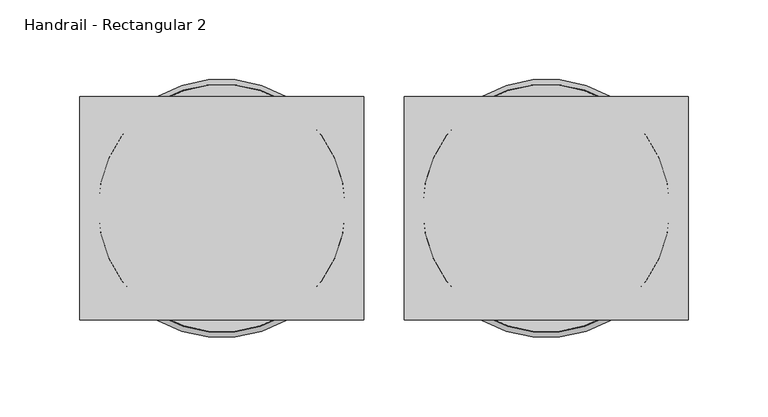
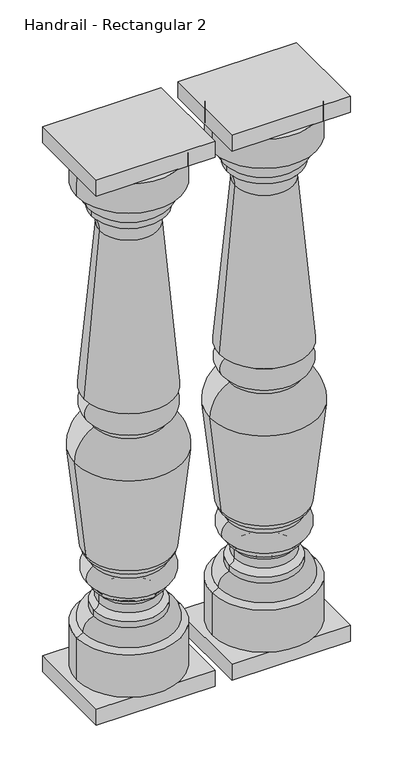
"""IFC4 building model written with IfcOpenShell, lengths in millimetres: railing geometry, Handrail - Rectangular 2."""

from ifc_helpers import new_model, si_unit, point, frame, origin, place, context, project, spatial, polyline, circle_curve, ellipse_curve, trimmed, outline, extrude, source, transform, mapped, element, save
from ifc_brep_helpers import plane_surface, cylinder_surface, revolved_surface, advanced_brep


def handrail_rectangular_2_7eab9a82(model_context):
    return source(origin(), model_context, "Body", "SolidModel", [
        advanced_brep(
        [(9255.6521895, -1691.0164768, 949.325), (9178.0909506, -1691.0164768, 949.325), (9333.2134284, -1691.0164768, 949.325), (9333.4396895, -1691.0164768, 136.525), (9177.8646895, -1691.0164768, 136.525), (9255.6521895, -1691.0164768, 136.525), (9333.4396895, -1691.0164768, 203.2), (9177.8646895, -1691.0164768, 203.2), (9323.8276556, -1691.0164768, 208.348485), (9187.4767235, -1691.0164768, 208.348485), (9308.0396895, -1691.0164768, 228.7310532), (9203.2646895, -1691.0164768, 228.7310532), (9308.0396895, -1691.0164768, 238.125), (9203.2646895, -1691.0164768, 238.125), (9300.4209727, -1691.0164768, 247.1598162), (9210.8834064, -1691.0164768, 247.1598162), (9300.4209727, -1691.0164768, 260.8401838), (9210.8834064, -1691.0164768, 260.8401838), (9308.0396895, -1691.0164768, 269.875), (9203.2646895, -1691.0164768, 269.875), (9308.0396895, -1691.0164768, 276.225), (9203.2646895, -1691.0164768, 276.225), (9308.8334395, -1691.0164768, 307.975), (9202.4709395, -1691.0164768, 307.975), (9308.8334395, -1691.0164768, 314.325), (9202.4709395, -1691.0164768, 314.325), (9319.6062243, -1691.0164768, 327.0157842), (9191.6981547, -1691.0164768, 327.0157842), (9336.693305, -1691.0164768, 481.3725887), (9174.6110741, -1691.0164768, 481.3725887), (9308.0396895, -1691.0164768, 528.6375), (9203.2646895, -1691.0164768, 528.6375), (9308.0396895, -1691.0164768, 534.9875), (9203.2646895, -1691.0164768, 534.9875), (9311.2146895, -1691.0164768, 569.9125), (9200.0896895, -1691.0164768, 569.9125), (9311.2146895, -1691.0164768, 573.0875), (9200.0896895, -1691.0164768, 573.0875), (9322.3271895, -1691.0164768, 577.85), (9188.9771895, -1691.0164768, 577.85), (9299.1486775, -1691.0164768, 836.3199218), (9212.1557016, -1691.0164768, 836.3199218), (9311.2146895, -1691.0164768, 863.6), (9200.0896895, -1691.0164768, 863.6), (9311.2146895, -1691.0164768, 873.125), (9200.0896895, -1691.0164768, 873.125), (9322.3271895, -1691.0164768, 900.1125), (9188.9771895, -1691.0164768, 900.1125), (9333.4396895, -1691.0164768, 903.2875), (9177.8646895, -1691.0164768, 903.2875)],
        [
            (0, 1),
            (1, 2, circle_curve(frame((9255.6521895, -1691.0164768, 949.325), z_axis=(0.0, 0.0, 1.0), x_axis=(-1.0, 0.0, 0.0)), 77.5612389)),
            (2, 0),
            (2, 1, circle_curve(frame((9255.6521895, -1691.0164768, 949.325), z_axis=(0.0, 0.0, 1.0), x_axis=(-1.0, 0.0, 0.0)), 77.5612389)),
            (3, 4, circle_curve(frame((9255.6521895, -1691.0164768, 136.525), z_axis=(0.0, 0.0, -1.0), x_axis=(-1.0, 0.0, 0.0)), 77.7875)),
            (4, 5),
            (5, 3),
            (4, 3, circle_curve(frame((9255.6521895, -1691.0164768, 136.525), z_axis=(0.0, 0.0, -1.0), x_axis=(-1.0, 0.0, 0.0)), 77.7875)),
            (6, 7, circle_curve(frame((9255.6521895, -1691.0164768, 203.2), z_axis=(0.0, 0.0, -1.0), x_axis=(-1.0, 0.0, 0.0)), 77.7875)),
            (7, 4),
            (3, 6),
            (7, 6, circle_curve(frame((9255.6521895, -1691.0164768, 203.2), z_axis=(0.0, 0.0, -1.0), x_axis=(-1.0, 0.0, 0.0)), 77.7875)),
            (8, 9, circle_curve(frame((9255.6521895, -1691.0164768, 208.348485), z_axis=(0.0, 0.0, -1.0), x_axis=(-1.0, 0.0, 0.0)), 68.175466)),
            (9, 7),
            (6, 8),
            (9, 8, circle_curve(frame((9255.6521895, -1691.0164768, 208.348485), z_axis=(0.0, 0.0, -1.0), x_axis=(-1.0, 0.0, 0.0)), 68.175466)),
            (10, 11, circle_curve(frame((9255.6521895, -1691.0164768, 228.7310532), z_axis=(0.0, 0.0, -1.0), x_axis=(-1.0, 0.0, 0.0)), 52.3875)),
            (11, 9, circle_curve(frame((9205.6397784, -1691.0164768, 210.5855331), z_axis=(0.0, -1.0, 0.0), x_axis=(1.0, 0.0, 0.0)), 18.3002991)),
            (8, 10, circle_curve(frame((9305.6646007, -1691.0164768, 210.5855331), z_axis=(0.0, -1.0, 0.0), x_axis=(-1.0, 0.0, 0.0)), 18.3002991)),
            (11, 10, circle_curve(frame((9255.6521895, -1691.0164768, 228.7310532), z_axis=(0.0, 0.0, -1.0), x_axis=(-1.0, 0.0, 0.0)), 52.3875)),
            (12, 13, circle_curve(frame((9255.6521895, -1691.0164768, 238.125), z_axis=(0.0, 0.0, -1.0), x_axis=(-1.0, 0.0, 0.0)), 52.3875)),
            (13, 11),
            (10, 12),
            (13, 12, circle_curve(frame((9255.6521895, -1691.0164768, 238.125), z_axis=(0.0, 0.0, -1.0), x_axis=(-1.0, 0.0, 0.0)), 52.3875)),
            (14, 15, circle_curve(frame((9255.6521895, -1691.0164768, 247.1598162), z_axis=(0.0, 0.0, -1.0), x_axis=(-1.0, 0.0, 0.0)), 44.7687831)),
            (15, 13, circle_curve(frame((9201.4793543, -1691.0164768, 247.3602005), z_axis=(0.0, 1.0, 0.0), x_axis=(1.0, 0.0, 0.0)), 9.4061868)),
            (12, 14, circle_curve(frame((9309.8250248, -1691.0164768, 247.3602005), z_axis=(0.0, 1.0, 0.0), x_axis=(-1.0, 0.0, 0.0)), 9.4061868)),
            (15, 14, circle_curve(frame((9255.6521895, -1691.0164768, 247.1598162), z_axis=(0.0, 0.0, -1.0), x_axis=(-1.0, 0.0, 0.0)), 44.7687831)),
            (16, 17, circle_curve(frame((9255.6521895, -1691.0164768, 260.8401838), z_axis=(0.0, 0.0, -1.0), x_axis=(-1.0, 0.0, 0.0)), 44.7687831)),
            (17, 15),
            (14, 16),
            (17, 16, circle_curve(frame((9255.6521895, -1691.0164768, 260.8401838), z_axis=(0.0, 0.0, -1.0), x_axis=(-1.0, 0.0, 0.0)), 44.7687831)),
            (18, 19, circle_curve(frame((9255.6521895, -1691.0164768, 269.875), z_axis=(0.0, 0.0, -1.0), x_axis=(-1.0, 0.0, 0.0)), 52.3875)),
            (19, 17, circle_curve(frame((9201.4793543, -1691.0164768, 260.6397995), z_axis=(0.0, 1.0, 0.0), x_axis=(1.0, 0.0, 0.0)), 9.4061868)),
            (16, 18, circle_curve(frame((9309.8250248, -1691.0164768, 260.6397995), z_axis=(0.0, 1.0, 0.0), x_axis=(-1.0, 0.0, 0.0)), 9.4061868)),
            (19, 18, circle_curve(frame((9255.6521895, -1691.0164768, 269.875), z_axis=(0.0, 0.0, -1.0), x_axis=(-1.0, 0.0, 0.0)), 52.3875)),
            (20, 21, circle_curve(frame((9255.6521895, -1691.0164768, 276.225), z_axis=(0.0, 0.0, -1.0), x_axis=(-1.0, 0.0, 0.0)), 52.3875)),
            (21, 19),
            (18, 20),
            (21, 20, circle_curve(frame((9255.6521895, -1691.0164768, 276.225), z_axis=(0.0, 0.0, -1.0), x_axis=(-1.0, 0.0, 0.0)), 52.3875)),
            (22, 23, circle_curve(frame((9255.6521895, -1691.0164768, 307.975), z_axis=(0.0, 0.0, -1.0), x_axis=(-1.0, 0.0, 0.0)), 53.18125)),
            (23, 21, circle_curve(frame((9208.8437772, -1691.0164768, 292.2493991), z_axis=(0.0, -1.0, 0.0), x_axis=(1.0, 0.0, 0.0)), 16.9678397)),
            (20, 22, circle_curve(frame((9302.4606019, -1691.0164768, 292.2493991), z_axis=(0.0, -1.0, 0.0), x_axis=(-1.0, 0.0, 0.0)), 16.9678397)),
            (23, 22, circle_curve(frame((9255.6521895, -1691.0164768, 307.975), z_axis=(0.0, 0.0, -1.0), x_axis=(-1.0, 0.0, 0.0)), 53.18125)),
            (24, 25, circle_curve(frame((9255.6521895, -1691.0164768, 314.325), z_axis=(0.0, 0.0, -1.0), x_axis=(-1.0, 0.0, 0.0)), 53.18125)),
            (25, 23),
            (22, 24),
            (25, 24, circle_curve(frame((9255.6521895, -1691.0164768, 314.325), z_axis=(0.0, 0.0, -1.0), x_axis=(-1.0, 0.0, 0.0)), 53.18125)),
            (26, 27, circle_curve(frame((9255.6521895, -1691.0164768, 327.0157842), z_axis=(0.0, 0.0, -1.0), x_axis=(-1.0, 0.0, 0.0)), 63.9540348)),
            (27, 25, circle_curve(frame((9212.304312, -1691.0164768, 333.5899445), z_axis=(0.0, -1.0, 0.0), x_axis=(1.0, 0.0, 0.0)), 21.6294545)),
            (24, 26, circle_curve(frame((9299.0000671, -1691.0164768, 333.5899445), z_axis=(0.0, -1.0, 0.0), x_axis=(-1.0, 0.0, 0.0)), 21.6294545)),
            (27, 26, circle_curve(frame((9255.6521895, -1691.0164768, 327.0157842), z_axis=(0.0, 0.0, -1.0), x_axis=(-1.0, 0.0, 0.0)), 63.9540348)),
            (28, 29, circle_curve(frame((9255.6521895, -1691.0164768, 481.3725887), z_axis=(0.0, 0.0, -1.0), x_axis=(-1.0, 0.0, 0.0)), 81.0411154)),
            (29, 27, circle_curve(frame((10668.9385198, -1691.0164768, 568.6683698), z_axis=(0.0, -1.0, 0.0), x_axis=(1.0, 0.0, 0.0)), 1496.8751012)),
            (26, 28, circle_curve(frame((7842.3658592, -1691.0164768, 568.6683698), z_axis=(0.0, -1.0, 0.0), x_axis=(-1.0, 0.0, 0.0)), 1496.8751012)),
            (29, 28, circle_curve(frame((9255.6521895, -1691.0164768, 481.3725887), z_axis=(0.0, 0.0, -1.0), x_axis=(-1.0, 0.0, 0.0)), 81.0411154)),
            (30, 31, circle_curve(frame((9255.6521895, -1691.0164768, 528.6375), z_axis=(0.0, 0.0, -1.0), x_axis=(-1.0, 0.0, 0.0)), 52.3875)),
            (31, 29, circle_curve(frame((9226.3638402, -1691.0164768, 482.3161407), z_axis=(0.0, -1.0, 0.0), x_axis=(1.0, 0.0, 0.0)), 51.7613668)),
            (28, 30, circle_curve(frame((9284.9405389, -1691.0164768, 482.3161407), z_axis=(0.0, -1.0, 0.0), x_axis=(-1.0, 0.0, 0.0)), 51.7613668)),
            (31, 30, circle_curve(frame((9255.6521895, -1691.0164768, 528.6375), z_axis=(0.0, 0.0, -1.0), x_axis=(-1.0, 0.0, 0.0)), 52.3875)),
            (32, 33, circle_curve(frame((9255.6521895, -1691.0164768, 534.9875), z_axis=(0.0, 0.0, -1.0), x_axis=(-1.0, 0.0, 0.0)), 52.3875)),
            (33, 31),
            (30, 32),
            (33, 32, circle_curve(frame((9255.6521895, -1691.0164768, 534.9875), z_axis=(0.0, 0.0, -1.0), x_axis=(-1.0, 0.0, 0.0)), 52.3875)),
            (34, 35, circle_curve(frame((9255.6521895, -1691.0164768, 569.9125), z_axis=(0.0, 0.0, -1.0), x_axis=(-1.0, 0.0, 0.0)), 55.5625)),
            (35, 33, circle_curve(frame((9208.3309419, -1691.0164768, 553.0548866), z_axis=(0.0, -1.0, 0.0), x_axis=(1.0, 0.0, 0.0)), 18.7642578)),
            (32, 34, circle_curve(frame((9302.9734372, -1691.0164768, 553.0548866), z_axis=(0.0, -1.0, 0.0), x_axis=(-1.0, 0.0, 0.0)), 18.7642578)),
            (35, 34, circle_curve(frame((9255.6521895, -1691.0164768, 569.9125), z_axis=(0.0, 0.0, -1.0), x_axis=(-1.0, 0.0, 0.0)), 55.5625)),
            (36, 37, circle_curve(frame((9255.6521895, -1691.0164768, 573.0875), z_axis=(0.0, 0.0, -1.0), x_axis=(-1.0, 0.0, 0.0)), 55.5625)),
            (37, 35),
            (34, 36),
            (37, 36, circle_curve(frame((9255.6521895, -1691.0164768, 573.0875), z_axis=(0.0, 0.0, -1.0), x_axis=(-1.0, 0.0, 0.0)), 55.5625)),
            (38, 39, circle_curve(frame((9255.6521895, -1691.0164768, 577.85), z_axis=(0.0, 0.0, -1.0), x_axis=(-1.0, 0.0, 0.0)), 66.675)),
            (39, 37),
            (36, 38),
            (39, 38, circle_curve(frame((9255.6521895, -1691.0164768, 577.85), z_axis=(0.0, 0.0, -1.0), x_axis=(-1.0, 0.0, 0.0)), 66.675)),
            (40, 41, circle_curve(frame((9255.6521895, -1691.0164768, 836.3199218), z_axis=(0.0, 0.0, -1.0), x_axis=(-1.0, 0.0, 0.0)), 43.4964879)),
            (41, 39, circle_curve(frame((7565.3192757, -1691.0164768, 853.7271544), z_axis=(0.0, 1.0, 0.0), x_axis=(1.0, 0.0, 0.0)), 1646.9284215)),
            (38, 40, circle_curve(frame((10945.9851034, -1691.0164768, 853.7271544), z_axis=(0.0, 1.0, 0.0), x_axis=(-1.0, 0.0, 0.0)), 1646.9284215)),
            (41, 40, circle_curve(frame((9255.6521895, -1691.0164768, 836.3199218), z_axis=(0.0, 0.0, -1.0), x_axis=(-1.0, 0.0, 0.0)), 43.4964879)),
            (42, 43, circle_curve(frame((9255.6521895, -1691.0164768, 863.6), z_axis=(0.0, 0.0, -1.0), x_axis=(-1.0, 0.0, 0.0)), 55.5625)),
            (43, 41, circle_curve(frame((9179.4515427, -1691.0164768, 838.1632773), z_axis=(0.0, 1.0, 0.0), x_axis=(1.0, 0.0, 0.0)), 32.7560676)),
            (40, 42, circle_curve(frame((9331.8528363, -1691.0164768, 838.1632773), z_axis=(0.0, 1.0, 0.0), x_axis=(-1.0, 0.0, 0.0)), 32.7560676)),
            (43, 42, circle_curve(frame((9255.6521895, -1691.0164768, 863.6), z_axis=(0.0, 0.0, -1.0), x_axis=(-1.0, 0.0, 0.0)), 55.5625)),
            (44, 45, circle_curve(frame((9255.6521895, -1691.0164768, 873.125), z_axis=(0.0, 0.0, -1.0), x_axis=(-1.0, 0.0, 0.0)), 55.5625)),
            (45, 43),
            (42, 44),
            (45, 44, circle_curve(frame((9255.6521895, -1691.0164768, 873.125), z_axis=(0.0, 0.0, -1.0), x_axis=(-1.0, 0.0, 0.0)), 55.5625)),
            (46, 47, circle_curve(frame((9255.6521895, -1691.0164768, 900.1125), z_axis=(0.0, 0.0, -1.0), x_axis=(-1.0, 0.0, 0.0)), 66.675)),
            (47, 45, circle_curve(frame((9218.3374113, -1691.0164768, 896.4203854), z_axis=(0.0, -1.0, 0.0), x_axis=(1.0, 0.0, 0.0)), 29.5914571)),
            (44, 46, circle_curve(frame((9292.9669678, -1691.0164768, 896.4203854), z_axis=(0.0, -1.0, 0.0), x_axis=(-1.0, 0.0, 0.0)), 29.5914571)),
            (47, 46, circle_curve(frame((9255.6521895, -1691.0164768, 900.1125), z_axis=(0.0, 0.0, -1.0), x_axis=(-1.0, 0.0, 0.0)), 66.675)),
            (48, 49, circle_curve(frame((9255.6521895, -1691.0164768, 903.2875), z_axis=(0.0, 0.0, -1.0), x_axis=(-1.0, 0.0, 0.0)), 77.7875)),
            (49, 47),
            (46, 48),
            (49, 48, circle_curve(frame((9255.6521895, -1691.0164768, 903.2875), z_axis=(0.0, 0.0, -1.0), x_axis=(-1.0, 0.0, 0.0)), 77.7875)),
            (1, 49),
            (48, 2),
        ],
        [
            plane_surface(frame((9255.6521895, -1691.0164768, 949.325), z_axis=(0.0, 0.0, 1.0), x_axis=(-1.0, 0.0, 0.0))),
            plane_surface(frame((9255.6521895, -1691.0164768, 136.525), z_axis=(0.0, 0.0, -1.0), x_axis=(-1.0, 0.0, 0.0))),
            cylinder_surface(frame((9255.6521895, -1691.0164768, 1019.175), z_axis=(0.0, 0.0, 1.0), x_axis=(-1.0, 0.0, 0.0)), 77.7875),
            revolved_surface(polyline([(9177.8646895, -1691.0164768, 203.2), (9187.4767235, -1691.0164768, 208.348485)]), (9255.6521895, -1691.0164768, 1019.175), (0.0, 0.0, 1.0)),
            revolved_surface(trimmed(ellipse_curve(frame((9205.6397784, -1691.0164768, 210.5855331), z_axis=(0.0, 1.0, 0.0), x_axis=(1.0, 0.0, 0.0)), 18.3002991, 18.3002991), [point((9187.4767235, -1691.0164768, 208.348485))], [point((9203.2646895, -1691.0164768, 228.7310532))], True, "CARTESIAN"), (9255.6521895, -1691.0164768, 1019.175), (0.0, 0.0, 1.0)),
            cylinder_surface(frame((9255.6521895, -1691.0164768, 1019.175), z_axis=(0.0, 0.0, 1.0), x_axis=(-1.0, 0.0, 0.0)), 52.3875),
            revolved_surface(trimmed(ellipse_curve(frame((9201.4793543, -1691.0164768, 247.3602005), z_axis=(0.0, -1.0, 0.0), x_axis=(1.0, 0.0, 0.0)), 9.4061868, 9.4061868), [point((9203.2646895, -1691.0164768, 238.125))], [point((9210.8834064, -1691.0164768, 247.1598162))], True, "CARTESIAN"), (9255.6521895, -1691.0164768, 1019.175), (0.0, 0.0, 1.0)),
            cylinder_surface(frame((9255.6521895, -1691.0164768, 1019.175), z_axis=(0.0, 0.0, 1.0), x_axis=(-1.0, 0.0, 0.0)), 44.7687831),
            revolved_surface(trimmed(ellipse_curve(frame((9201.4793543, -1691.0164768, 260.6397995), z_axis=(0.0, -1.0, 0.0), x_axis=(1.0, 0.0, 0.0)), 9.4061868, 9.4061868), [point((9210.8834064, -1691.0164768, 260.8401838))], [point((9203.2646895, -1691.0164768, 269.875))], True, "CARTESIAN"), (9255.6521895, -1691.0164768, 1019.175), (0.0, 0.0, 1.0)),
            revolved_surface(trimmed(ellipse_curve(frame((9208.8437772, -1691.0164768, 292.2493991), z_axis=(0.0, 1.0, 0.0), x_axis=(1.0, 0.0, 0.0)), 16.9678397, 16.9678397), [point((9203.2646895, -1691.0164768, 276.225))], [point((9202.4709395, -1691.0164768, 307.975))], True, "CARTESIAN"), (9255.6521895, -1691.0164768, 1019.175), (0.0, 0.0, 1.0)),
            cylinder_surface(frame((9255.6521895, -1691.0164768, 1019.175), z_axis=(0.0, 0.0, 1.0), x_axis=(-1.0, 0.0, 0.0)), 53.18125),
            revolved_surface(trimmed(ellipse_curve(frame((9212.304312, -1691.0164768, 333.5899445), z_axis=(0.0, 1.0, 0.0), x_axis=(1.0, 0.0, 0.0)), 21.6294545, 21.6294545), [point((9202.4709395, -1691.0164768, 314.325))], [point((9191.6981547, -1691.0164768, 327.0157842))], True, "CARTESIAN"), (9255.6521895, -1691.0164768, 1019.175), (0.0, 0.0, 1.0)),
            revolved_surface(trimmed(ellipse_curve(frame((10668.9385198, -1691.0164768, 568.6683698), z_axis=(0.0, 1.0, 0.0), x_axis=(1.0, 0.0, 0.0)), 1496.8751012, 1496.8751012), [point((9191.6981547, -1691.0164768, 327.0157842))], [point((9174.6110741, -1691.0164768, 481.3725887))], True, "CARTESIAN"), (9255.6521895, -1691.0164768, 1019.175), (0.0, 0.0, 1.0)),
            revolved_surface(trimmed(ellipse_curve(frame((9226.3638402, -1691.0164768, 482.3161407), z_axis=(0.0, 1.0, 0.0), x_axis=(1.0, 0.0, 0.0)), 51.7613668, 51.7613668), [point((9174.6110741, -1691.0164768, 481.3725887))], [point((9203.2646895, -1691.0164768, 528.6375))], True, "CARTESIAN"), (9255.6521895, -1691.0164768, 1019.175), (0.0, 0.0, 1.0)),
            revolved_surface(trimmed(ellipse_curve(frame((9208.3309419, -1691.0164768, 553.0548866), z_axis=(0.0, 1.0, 0.0), x_axis=(1.0, 0.0, 0.0)), 18.7642578, 18.7642578), [point((9203.2646895, -1691.0164768, 534.9875))], [point((9200.0896895, -1691.0164768, 569.9125))], True, "CARTESIAN"), (9255.6521895, -1691.0164768, 1019.175), (0.0, 0.0, 1.0)),
            cylinder_surface(frame((9255.6521895, -1691.0164768, 1019.175), z_axis=(0.0, 0.0, 1.0), x_axis=(-1.0, 0.0, 0.0)), 55.5625),
            revolved_surface(polyline([(9200.0896895, -1691.0164768, 573.0875), (9188.9771895, -1691.0164768, 577.85)]), (9255.6521895, -1691.0164768, 1019.175), (0.0, 0.0, 1.0)),
            revolved_surface(trimmed(ellipse_curve(frame((7565.3192757, -1691.0164768, 853.7271544), z_axis=(0.0, -1.0, 0.0), x_axis=(1.0, 0.0, 0.0)), 1646.9284215, 1646.9284215), [point((9188.9771895, -1691.0164768, 577.85))], [point((9212.1557016, -1691.0164768, 836.3199218))], True, "CARTESIAN"), (9255.6521895, -1691.0164768, 1019.175), (0.0, 0.0, 1.0)),
            revolved_surface(trimmed(ellipse_curve(frame((9179.4515427, -1691.0164768, 838.1632773), z_axis=(0.0, -1.0, 0.0), x_axis=(1.0, 0.0, 0.0)), 32.7560676, 32.7560676), [point((9212.1557016, -1691.0164768, 836.3199218))], [point((9200.0896895, -1691.0164768, 863.6))], True, "CARTESIAN"), (9255.6521895, -1691.0164768, 1019.175), (0.0, 0.0, 1.0)),
            revolved_surface(trimmed(ellipse_curve(frame((9218.3374113, -1691.0164768, 896.4203854), z_axis=(0.0, 1.0, 0.0), x_axis=(1.0, 0.0, 0.0)), 29.5914571, 29.5914571), [point((9200.0896895, -1691.0164768, 873.125))], [point((9188.9771895, -1691.0164768, 900.1125))], True, "CARTESIAN"), (9255.6521895, -1691.0164768, 1019.175), (0.0, 0.0, 1.0)),
            revolved_surface(polyline([(9188.9771895, -1691.0164768, 900.1125), (9177.8646895, -1691.0164768, 903.2875)]), (9255.6521895, -1691.0164768, 1019.175), (0.0, 0.0, 1.0)),
            revolved_surface(polyline([(9177.8646895, -1691.0164768, 903.2875), (9178.0909506, -1691.0164768, 949.325)]), (9255.6521895, -1691.0164768, 1019.175), (0.0, 0.0, 1.0)),
        ],
        [
            (0, [[1, 2, 3]]),
            (0, [[-3, 4, -1]]),
            (1, [[5, 6, 7]]),
            (1, [[8, -7, -6]]),
            (2, [[9, 10, -5, 11]]),
            (2, [[12, -11, -8, -10]]),
            (3, [[13, 14, -9, 15]]),
            (3, [[16, -15, -12, -14]]),
            (4, [[17, 18, -13, 19]]),
            (4, [[20, -19, -16, -18]]),
            (5, [[21, 22, -17, 23]]),
            (5, [[24, -23, -20, -22]]),
            (6, [[25, 26, -21, 27]]),
            (6, [[28, -27, -24, -26]]),
            (7, [[29, 30, -25, 31]]),
            (7, [[32, -31, -28, -30]]),
            (8, [[33, 34, -29, 35]]),
            (8, [[36, -35, -32, -34]]),
            (5, [[37, 38, -33, 39]]),
            (5, [[40, -39, -36, -38]]),
            (9, [[41, 42, -37, 43]]),
            (9, [[44, -43, -40, -42]]),
            (10, [[45, 46, -41, 47]]),
            (10, [[48, -47, -44, -46]]),
            (11, [[49, 50, -45, 51]]),
            (11, [[52, -51, -48, -50]]),
            (12, [[53, 54, -49, 55]]),
            (12, [[56, -55, -52, -54]]),
            (13, [[57, 58, -53, 59]]),
            (13, [[60, -59, -56, -58]]),
            (5, [[61, 62, -57, 63]]),
            (5, [[64, -63, -60, -62]]),
            (14, [[65, 66, -61, 67]]),
            (14, [[68, -67, -64, -66]]),
            (15, [[69, 70, -65, 71]]),
            (15, [[72, -71, -68, -70]]),
            (16, [[73, 74, -69, 75]]),
            (16, [[76, -75, -72, -74]]),
            (17, [[77, 78, -73, 79]]),
            (17, [[80, -79, -76, -78]]),
            (18, [[81, 82, -77, 83]]),
            (18, [[84, -83, -80, -82]]),
            (15, [[85, 86, -81, 87]]),
            (15, [[88, -87, -84, -86]]),
            (19, [[89, 90, -85, 91]]),
            (19, [[92, -91, -88, -90]]),
            (20, [[93, 94, -89, 95]]),
            (20, [[96, -95, -92, -94]]),
            (21, [[-2, 97, -93, 98]]),
            (21, [[-4, -98, -96, -97]]),
        ],
    ),
        extrude(outline(polyline([(9166.7521895, -1760.8664768), (9166.7521895, -1621.1664768), (9344.5521895, -1621.1664768), (9344.5521895, -1760.8664768), (9166.7521895, -1760.8664768)])), frame((0.0, 0.0, 111.125), z_axis=(0.0, 0.0, 1.0), x_axis=(1.0, 0.0, 0.0)), (0.0, 0.0, 1.0), 25.4),
        extrude(outline(polyline([(9166.7521895, -1621.1664768), (9344.5521895, -1621.1664768), (9344.5521895, -1760.8664768), (9166.7521895, -1760.8664768), (9166.7521895, -1621.1664768)])), frame((0.0, 0.0, 949.325), z_axis=(0.0, 0.0, 1.0), x_axis=(1.0, 0.0, 0.0)), (0.0, 0.0, 1.0), 25.4),
        advanced_brep(
        [(9052.4521895, -1691.0164768, 949.325), (8974.8909506, -1691.0164768, 949.325), (9130.0134284, -1691.0164768, 949.325), (9130.2396895, -1691.0164768, 136.525), (8974.6646895, -1691.0164768, 136.525), (9052.4521895, -1691.0164768, 136.525), (9130.2396895, -1691.0164768, 203.2), (8974.6646895, -1691.0164768, 203.2), (9120.6276556, -1691.0164768, 208.348485), (8984.2767235, -1691.0164768, 208.348485), (9104.8396895, -1691.0164768, 228.7310532), (9000.0646895, -1691.0164768, 228.7310532), (9104.8396895, -1691.0164768, 238.125), (9000.0646895, -1691.0164768, 238.125), (9097.2209727, -1691.0164768, 247.1598162), (9007.6834064, -1691.0164768, 247.1598162), (9097.2209727, -1691.0164768, 260.8401838), (9007.6834064, -1691.0164768, 260.8401838), (9104.8396895, -1691.0164768, 269.875), (9000.0646895, -1691.0164768, 269.875), (9104.8396895, -1691.0164768, 276.225), (9000.0646895, -1691.0164768, 276.225), (9105.6334395, -1691.0164768, 307.975), (8999.2709395, -1691.0164768, 307.975), (9105.6334395, -1691.0164768, 314.325), (8999.2709395, -1691.0164768, 314.325), (9116.4062243, -1691.0164768, 327.0157842), (8988.4981547, -1691.0164768, 327.0157842), (9133.493305, -1691.0164768, 481.3725887), (8971.4110741, -1691.0164768, 481.3725887), (9104.8396895, -1691.0164768, 528.6375), (9000.0646895, -1691.0164768, 528.6375), (9104.8396895, -1691.0164768, 534.9875), (9000.0646895, -1691.0164768, 534.9875), (9108.0146895, -1691.0164768, 569.9125), (8996.8896895, -1691.0164768, 569.9125), (9108.0146895, -1691.0164768, 573.0875), (8996.8896895, -1691.0164768, 573.0875), (9119.1271895, -1691.0164768, 577.85), (8985.7771895, -1691.0164768, 577.85), (9095.9486775, -1691.0164768, 836.3199218), (9008.9557016, -1691.0164768, 836.3199218), (9108.0146895, -1691.0164768, 863.6), (8996.8896895, -1691.0164768, 863.6), (9108.0146895, -1691.0164768, 873.125), (8996.8896895, -1691.0164768, 873.125), (9119.1271895, -1691.0164768, 900.1125), (8985.7771895, -1691.0164768, 900.1125), (9130.2396895, -1691.0164768, 903.2875), (8974.6646895, -1691.0164768, 903.2875)],
        [
            (0, 1),
            (1, 2, circle_curve(frame((9052.4521895, -1691.0164768, 949.325), z_axis=(0.0, 0.0, 1.0), x_axis=(-1.0, 0.0, 0.0)), 77.5612389)),
            (2, 0),
            (2, 1, circle_curve(frame((9052.4521895, -1691.0164768, 949.325), z_axis=(0.0, 0.0, 1.0), x_axis=(-1.0, 0.0, 0.0)), 77.5612389)),
            (3, 4, circle_curve(frame((9052.4521895, -1691.0164768, 136.525), z_axis=(0.0, 0.0, -1.0), x_axis=(-1.0, 0.0, 0.0)), 77.7875)),
            (4, 5),
            (5, 3),
            (4, 3, circle_curve(frame((9052.4521895, -1691.0164768, 136.525), z_axis=(0.0, 0.0, -1.0), x_axis=(-1.0, 0.0, 0.0)), 77.7875)),
            (6, 7, circle_curve(frame((9052.4521895, -1691.0164768, 203.2), z_axis=(0.0, 0.0, -1.0), x_axis=(-1.0, 0.0, 0.0)), 77.7875)),
            (7, 4),
            (3, 6),
            (7, 6, circle_curve(frame((9052.4521895, -1691.0164768, 203.2), z_axis=(0.0, 0.0, -1.0), x_axis=(-1.0, 0.0, 0.0)), 77.7875)),
            (8, 9, circle_curve(frame((9052.4521895, -1691.0164768, 208.348485), z_axis=(0.0, 0.0, -1.0), x_axis=(-1.0, 0.0, 0.0)), 68.175466)),
            (9, 7),
            (6, 8),
            (9, 8, circle_curve(frame((9052.4521895, -1691.0164768, 208.348485), z_axis=(0.0, 0.0, -1.0), x_axis=(-1.0, 0.0, 0.0)), 68.175466)),
            (10, 11, circle_curve(frame((9052.4521895, -1691.0164768, 228.7310532), z_axis=(0.0, 0.0, -1.0), x_axis=(-1.0, 0.0, 0.0)), 52.3875)),
            (11, 9, circle_curve(frame((9002.4397784, -1691.0164768, 210.5855331), z_axis=(0.0, -1.0, 0.0), x_axis=(1.0, 0.0, 0.0)), 18.3002991)),
            (8, 10, circle_curve(frame((9102.4646007, -1691.0164768, 210.5855331), z_axis=(0.0, -1.0, 0.0), x_axis=(-1.0, 0.0, 0.0)), 18.3002991)),
            (11, 10, circle_curve(frame((9052.4521895, -1691.0164768, 228.7310532), z_axis=(0.0, 0.0, -1.0), x_axis=(-1.0, 0.0, 0.0)), 52.3875)),
            (12, 13, circle_curve(frame((9052.4521895, -1691.0164768, 238.125), z_axis=(0.0, 0.0, -1.0), x_axis=(-1.0, 0.0, 0.0)), 52.3875)),
            (13, 11),
            (10, 12),
            (13, 12, circle_curve(frame((9052.4521895, -1691.0164768, 238.125), z_axis=(0.0, 0.0, -1.0), x_axis=(-1.0, 0.0, 0.0)), 52.3875)),
            (14, 15, circle_curve(frame((9052.4521895, -1691.0164768, 247.1598162), z_axis=(0.0, 0.0, -1.0), x_axis=(-1.0, 0.0, 0.0)), 44.7687831)),
            (15, 13, circle_curve(frame((8998.2793543, -1691.0164768, 247.3602005), z_axis=(0.0, 1.0, 0.0), x_axis=(1.0, 0.0, 0.0)), 9.4061868)),
            (12, 14, circle_curve(frame((9106.6250248, -1691.0164768, 247.3602005), z_axis=(0.0, 1.0, 0.0), x_axis=(-1.0, 0.0, 0.0)), 9.4061868)),
            (15, 14, circle_curve(frame((9052.4521895, -1691.0164768, 247.1598162), z_axis=(0.0, 0.0, -1.0), x_axis=(-1.0, 0.0, 0.0)), 44.7687831)),
            (16, 17, circle_curve(frame((9052.4521895, -1691.0164768, 260.8401838), z_axis=(0.0, 0.0, -1.0), x_axis=(-1.0, 0.0, 0.0)), 44.7687831)),
            (17, 15),
            (14, 16),
            (17, 16, circle_curve(frame((9052.4521895, -1691.0164768, 260.8401838), z_axis=(0.0, 0.0, -1.0), x_axis=(-1.0, 0.0, 0.0)), 44.7687831)),
            (18, 19, circle_curve(frame((9052.4521895, -1691.0164768, 269.875), z_axis=(0.0, 0.0, -1.0), x_axis=(-1.0, 0.0, 0.0)), 52.3875)),
            (19, 17, circle_curve(frame((8998.2793543, -1691.0164768, 260.6397995), z_axis=(0.0, 1.0, 0.0), x_axis=(1.0, 0.0, 0.0)), 9.4061868)),
            (16, 18, circle_curve(frame((9106.6250248, -1691.0164768, 260.6397995), z_axis=(0.0, 1.0, 0.0), x_axis=(-1.0, 0.0, 0.0)), 9.4061868)),
            (19, 18, circle_curve(frame((9052.4521895, -1691.0164768, 269.875), z_axis=(0.0, 0.0, -1.0), x_axis=(-1.0, 0.0, 0.0)), 52.3875)),
            (20, 21, circle_curve(frame((9052.4521895, -1691.0164768, 276.225), z_axis=(0.0, 0.0, -1.0), x_axis=(-1.0, 0.0, 0.0)), 52.3875)),
            (21, 19),
            (18, 20),
            (21, 20, circle_curve(frame((9052.4521895, -1691.0164768, 276.225), z_axis=(0.0, 0.0, -1.0), x_axis=(-1.0, 0.0, 0.0)), 52.3875)),
            (22, 23, circle_curve(frame((9052.4521895, -1691.0164768, 307.975), z_axis=(0.0, 0.0, -1.0), x_axis=(-1.0, 0.0, 0.0)), 53.18125)),
            (23, 21, circle_curve(frame((9005.6437772, -1691.0164768, 292.2493991), z_axis=(0.0, -1.0, 0.0), x_axis=(1.0, 0.0, 0.0)), 16.9678397)),
            (20, 22, circle_curve(frame((9099.2606019, -1691.0164768, 292.2493991), z_axis=(0.0, -1.0, 0.0), x_axis=(-1.0, 0.0, 0.0)), 16.9678397)),
            (23, 22, circle_curve(frame((9052.4521895, -1691.0164768, 307.975), z_axis=(0.0, 0.0, -1.0), x_axis=(-1.0, 0.0, 0.0)), 53.18125)),
            (24, 25, circle_curve(frame((9052.4521895, -1691.0164768, 314.325), z_axis=(0.0, 0.0, -1.0), x_axis=(-1.0, 0.0, 0.0)), 53.18125)),
            (25, 23),
            (22, 24),
            (25, 24, circle_curve(frame((9052.4521895, -1691.0164768, 314.325), z_axis=(0.0, 0.0, -1.0), x_axis=(-1.0, 0.0, 0.0)), 53.18125)),
            (26, 27, circle_curve(frame((9052.4521895, -1691.0164768, 327.0157842), z_axis=(0.0, 0.0, -1.0), x_axis=(-1.0, 0.0, 0.0)), 63.9540348)),
            (27, 25, circle_curve(frame((9009.104312, -1691.0164768, 333.5899445), z_axis=(0.0, -1.0, 0.0), x_axis=(1.0, 0.0, 0.0)), 21.6294545)),
            (24, 26, circle_curve(frame((9095.8000671, -1691.0164768, 333.5899445), z_axis=(0.0, -1.0, 0.0), x_axis=(-1.0, 0.0, 0.0)), 21.6294545)),
            (27, 26, circle_curve(frame((9052.4521895, -1691.0164768, 327.0157842), z_axis=(0.0, 0.0, -1.0), x_axis=(-1.0, 0.0, 0.0)), 63.9540348)),
            (28, 29, circle_curve(frame((9052.4521895, -1691.0164768, 481.3725887), z_axis=(0.0, 0.0, -1.0), x_axis=(-1.0, 0.0, 0.0)), 81.0411154)),
            (29, 27, circle_curve(frame((10465.7385198, -1691.0164768, 568.6683698), z_axis=(0.0, -1.0, 0.0), x_axis=(1.0, 0.0, 0.0)), 1496.8751012)),
            (26, 28, circle_curve(frame((7639.1658592, -1691.0164768, 568.6683698), z_axis=(0.0, -1.0, 0.0), x_axis=(-1.0, 0.0, 0.0)), 1496.8751012)),
            (29, 28, circle_curve(frame((9052.4521895, -1691.0164768, 481.3725887), z_axis=(0.0, 0.0, -1.0), x_axis=(-1.0, 0.0, 0.0)), 81.0411154)),
            (30, 31, circle_curve(frame((9052.4521895, -1691.0164768, 528.6375), z_axis=(0.0, 0.0, -1.0), x_axis=(-1.0, 0.0, 0.0)), 52.3875)),
            (31, 29, circle_curve(frame((9023.1638402, -1691.0164768, 482.3161407), z_axis=(0.0, -1.0, 0.0), x_axis=(1.0, 0.0, 0.0)), 51.7613668)),
            (28, 30, circle_curve(frame((9081.7405389, -1691.0164768, 482.3161407), z_axis=(0.0, -1.0, 0.0), x_axis=(-1.0, 0.0, 0.0)), 51.7613668)),
            (31, 30, circle_curve(frame((9052.4521895, -1691.0164768, 528.6375), z_axis=(0.0, 0.0, -1.0), x_axis=(-1.0, 0.0, 0.0)), 52.3875)),
            (32, 33, circle_curve(frame((9052.4521895, -1691.0164768, 534.9875), z_axis=(0.0, 0.0, -1.0), x_axis=(-1.0, 0.0, 0.0)), 52.3875)),
            (33, 31),
            (30, 32),
            (33, 32, circle_curve(frame((9052.4521895, -1691.0164768, 534.9875), z_axis=(0.0, 0.0, -1.0), x_axis=(-1.0, 0.0, 0.0)), 52.3875)),
            (34, 35, circle_curve(frame((9052.4521895, -1691.0164768, 569.9125), z_axis=(0.0, 0.0, -1.0), x_axis=(-1.0, 0.0, 0.0)), 55.5625)),
            (35, 33, circle_curve(frame((9005.1309419, -1691.0164768, 553.0548866), z_axis=(0.0, -1.0, 0.0), x_axis=(1.0, 0.0, 0.0)), 18.7642578)),
            (32, 34, circle_curve(frame((9099.7734372, -1691.0164768, 553.0548866), z_axis=(0.0, -1.0, 0.0), x_axis=(-1.0, 0.0, 0.0)), 18.7642578)),
            (35, 34, circle_curve(frame((9052.4521895, -1691.0164768, 569.9125), z_axis=(0.0, 0.0, -1.0), x_axis=(-1.0, 0.0, 0.0)), 55.5625)),
            (36, 37, circle_curve(frame((9052.4521895, -1691.0164768, 573.0875), z_axis=(0.0, 0.0, -1.0), x_axis=(-1.0, 0.0, 0.0)), 55.5625)),
            (37, 35),
            (34, 36),
            (37, 36, circle_curve(frame((9052.4521895, -1691.0164768, 573.0875), z_axis=(0.0, 0.0, -1.0), x_axis=(-1.0, 0.0, 0.0)), 55.5625)),
            (38, 39, circle_curve(frame((9052.4521895, -1691.0164768, 577.85), z_axis=(0.0, 0.0, -1.0), x_axis=(-1.0, 0.0, 0.0)), 66.675)),
            (39, 37),
            (36, 38),
            (39, 38, circle_curve(frame((9052.4521895, -1691.0164768, 577.85), z_axis=(0.0, 0.0, -1.0), x_axis=(-1.0, 0.0, 0.0)), 66.675)),
            (40, 41, circle_curve(frame((9052.4521895, -1691.0164768, 836.3199218), z_axis=(0.0, 0.0, -1.0), x_axis=(-1.0, 0.0, 0.0)), 43.4964879)),
            (41, 39, circle_curve(frame((7362.1192757, -1691.0164768, 853.7271544), z_axis=(0.0, 1.0, 0.0), x_axis=(1.0, 0.0, 0.0)), 1646.9284215)),
            (38, 40, circle_curve(frame((10742.7851034, -1691.0164768, 853.7271544), z_axis=(0.0, 1.0, 0.0), x_axis=(-1.0, 0.0, 0.0)), 1646.9284215)),
            (41, 40, circle_curve(frame((9052.4521895, -1691.0164768, 836.3199218), z_axis=(0.0, 0.0, -1.0), x_axis=(-1.0, 0.0, 0.0)), 43.4964879)),
            (42, 43, circle_curve(frame((9052.4521895, -1691.0164768, 863.6), z_axis=(0.0, 0.0, -1.0), x_axis=(-1.0, 0.0, 0.0)), 55.5625)),
            (43, 41, circle_curve(frame((8976.2515427, -1691.0164768, 838.1632773), z_axis=(0.0, 1.0, 0.0), x_axis=(1.0, 0.0, 0.0)), 32.7560676)),
            (40, 42, circle_curve(frame((9128.6528363, -1691.0164768, 838.1632773), z_axis=(0.0, 1.0, 0.0), x_axis=(-1.0, 0.0, 0.0)), 32.7560676)),
            (43, 42, circle_curve(frame((9052.4521895, -1691.0164768, 863.6), z_axis=(0.0, 0.0, -1.0), x_axis=(-1.0, 0.0, 0.0)), 55.5625)),
            (44, 45, circle_curve(frame((9052.4521895, -1691.0164768, 873.125), z_axis=(0.0, 0.0, -1.0), x_axis=(-1.0, 0.0, 0.0)), 55.5625)),
            (45, 43),
            (42, 44),
            (45, 44, circle_curve(frame((9052.4521895, -1691.0164768, 873.125), z_axis=(0.0, 0.0, -1.0), x_axis=(-1.0, 0.0, 0.0)), 55.5625)),
            (46, 47, circle_curve(frame((9052.4521895, -1691.0164768, 900.1125), z_axis=(0.0, 0.0, -1.0), x_axis=(-1.0, 0.0, 0.0)), 66.675)),
            (47, 45, circle_curve(frame((9015.1374113, -1691.0164768, 896.4203854), z_axis=(0.0, -1.0, 0.0), x_axis=(1.0, 0.0, 0.0)), 29.5914571)),
            (44, 46, circle_curve(frame((9089.7669678, -1691.0164768, 896.4203854), z_axis=(0.0, -1.0, 0.0), x_axis=(-1.0, 0.0, 0.0)), 29.5914571)),
            (47, 46, circle_curve(frame((9052.4521895, -1691.0164768, 900.1125), z_axis=(0.0, 0.0, -1.0), x_axis=(-1.0, 0.0, 0.0)), 66.675)),
            (48, 49, circle_curve(frame((9052.4521895, -1691.0164768, 903.2875), z_axis=(0.0, 0.0, -1.0), x_axis=(-1.0, 0.0, 0.0)), 77.7875)),
            (49, 47),
            (46, 48),
            (49, 48, circle_curve(frame((9052.4521895, -1691.0164768, 903.2875), z_axis=(0.0, 0.0, -1.0), x_axis=(-1.0, 0.0, 0.0)), 77.7875)),
            (1, 49),
            (48, 2),
        ],
        [
            plane_surface(frame((9052.4521895, -1691.0164768, 949.325), z_axis=(0.0, 0.0, 1.0), x_axis=(-1.0, 0.0, 0.0))),
            plane_surface(frame((9052.4521895, -1691.0164768, 136.525), z_axis=(0.0, 0.0, -1.0), x_axis=(-1.0, 0.0, 0.0))),
            cylinder_surface(frame((9052.4521895, -1691.0164768, 1019.175), z_axis=(0.0, 0.0, 1.0), x_axis=(-1.0, 0.0, 0.0)), 77.7875),
            revolved_surface(polyline([(8974.6646895, -1691.0164768, 203.2), (8984.2767235, -1691.0164768, 208.348485)]), (9052.4521895, -1691.0164768, 1019.175), (0.0, 0.0, 1.0)),
            revolved_surface(trimmed(ellipse_curve(frame((9002.4397784, -1691.0164768, 210.5855331), z_axis=(0.0, 1.0, 0.0), x_axis=(1.0, 0.0, 0.0)), 18.3002991, 18.3002991), [point((8984.2767235, -1691.0164768, 208.348485))], [point((9000.0646895, -1691.0164768, 228.7310532))], True, "CARTESIAN"), (9052.4521895, -1691.0164768, 1019.175), (0.0, 0.0, 1.0)),
            cylinder_surface(frame((9052.4521895, -1691.0164768, 1019.175), z_axis=(0.0, 0.0, 1.0), x_axis=(-1.0, 0.0, 0.0)), 52.3875),
            revolved_surface(trimmed(ellipse_curve(frame((8998.2793543, -1691.0164768, 247.3602005), z_axis=(0.0, -1.0, 0.0), x_axis=(1.0, 0.0, 0.0)), 9.4061868, 9.4061868), [point((9000.0646895, -1691.0164768, 238.125))], [point((9007.6834064, -1691.0164768, 247.1598162))], True, "CARTESIAN"), (9052.4521895, -1691.0164768, 1019.175), (0.0, 0.0, 1.0)),
            cylinder_surface(frame((9052.4521895, -1691.0164768, 1019.175), z_axis=(0.0, 0.0, 1.0), x_axis=(-1.0, 0.0, 0.0)), 44.7687831),
            revolved_surface(trimmed(ellipse_curve(frame((8998.2793543, -1691.0164768, 260.6397995), z_axis=(0.0, -1.0, 0.0), x_axis=(1.0, 0.0, 0.0)), 9.4061868, 9.4061868), [point((9007.6834064, -1691.0164768, 260.8401838))], [point((9000.0646895, -1691.0164768, 269.875))], True, "CARTESIAN"), (9052.4521895, -1691.0164768, 1019.175), (0.0, 0.0, 1.0)),
            revolved_surface(trimmed(ellipse_curve(frame((9005.6437772, -1691.0164768, 292.2493991), z_axis=(0.0, 1.0, 0.0), x_axis=(1.0, 0.0, 0.0)), 16.9678397, 16.9678397), [point((9000.0646895, -1691.0164768, 276.225))], [point((8999.2709395, -1691.0164768, 307.975))], True, "CARTESIAN"), (9052.4521895, -1691.0164768, 1019.175), (0.0, 0.0, 1.0)),
            cylinder_surface(frame((9052.4521895, -1691.0164768, 1019.175), z_axis=(0.0, 0.0, 1.0), x_axis=(-1.0, 0.0, 0.0)), 53.18125),
            revolved_surface(trimmed(ellipse_curve(frame((9009.104312, -1691.0164768, 333.5899445), z_axis=(0.0, 1.0, 0.0), x_axis=(1.0, 0.0, 0.0)), 21.6294545, 21.6294545), [point((8999.2709395, -1691.0164768, 314.325))], [point((8988.4981547, -1691.0164768, 327.0157842))], True, "CARTESIAN"), (9052.4521895, -1691.0164768, 1019.175), (0.0, 0.0, 1.0)),
            revolved_surface(trimmed(ellipse_curve(frame((10465.7385198, -1691.0164768, 568.6683698), z_axis=(0.0, 1.0, 0.0), x_axis=(1.0, 0.0, 0.0)), 1496.8751012, 1496.8751012), [point((8988.4981547, -1691.0164768, 327.0157842))], [point((8971.4110741, -1691.0164768, 481.3725887))], True, "CARTESIAN"), (9052.4521895, -1691.0164768, 1019.175), (0.0, 0.0, 1.0)),
            revolved_surface(trimmed(ellipse_curve(frame((9023.1638402, -1691.0164768, 482.3161407), z_axis=(0.0, 1.0, 0.0), x_axis=(1.0, 0.0, 0.0)), 51.7613668, 51.7613668), [point((8971.4110741, -1691.0164768, 481.3725887))], [point((9000.0646895, -1691.0164768, 528.6375))], True, "CARTESIAN"), (9052.4521895, -1691.0164768, 1019.175), (0.0, 0.0, 1.0)),
            revolved_surface(trimmed(ellipse_curve(frame((9005.1309419, -1691.0164768, 553.0548866), z_axis=(0.0, 1.0, 0.0), x_axis=(1.0, 0.0, 0.0)), 18.7642578, 18.7642578), [point((9000.0646895, -1691.0164768, 534.9875))], [point((8996.8896895, -1691.0164768, 569.9125))], True, "CARTESIAN"), (9052.4521895, -1691.0164768, 1019.175), (0.0, 0.0, 1.0)),
            cylinder_surface(frame((9052.4521895, -1691.0164768, 1019.175), z_axis=(0.0, 0.0, 1.0), x_axis=(-1.0, 0.0, 0.0)), 55.5625),
            revolved_surface(polyline([(8996.8896895, -1691.0164768, 573.0875), (8985.7771895, -1691.0164768, 577.85)]), (9052.4521895, -1691.0164768, 1019.175), (0.0, 0.0, 1.0)),
            revolved_surface(trimmed(ellipse_curve(frame((7362.1192757, -1691.0164768, 853.7271544), z_axis=(0.0, -1.0, 0.0), x_axis=(1.0, 0.0, 0.0)), 1646.9284215, 1646.9284215), [point((8985.7771895, -1691.0164768, 577.85))], [point((9008.9557016, -1691.0164768, 836.3199218))], True, "CARTESIAN"), (9052.4521895, -1691.0164768, 1019.175), (0.0, 0.0, 1.0)),
            revolved_surface(trimmed(ellipse_curve(frame((8976.2515427, -1691.0164768, 838.1632773), z_axis=(0.0, -1.0, 0.0), x_axis=(1.0, 0.0, 0.0)), 32.7560676, 32.7560676), [point((9008.9557016, -1691.0164768, 836.3199218))], [point((8996.8896895, -1691.0164768, 863.6))], True, "CARTESIAN"), (9052.4521895, -1691.0164768, 1019.175), (0.0, 0.0, 1.0)),
            revolved_surface(trimmed(ellipse_curve(frame((9015.1374113, -1691.0164768, 896.4203854), z_axis=(0.0, 1.0, 0.0), x_axis=(1.0, 0.0, 0.0)), 29.5914571, 29.5914571), [point((8996.8896895, -1691.0164768, 873.125))], [point((8985.7771895, -1691.0164768, 900.1125))], True, "CARTESIAN"), (9052.4521895, -1691.0164768, 1019.175), (0.0, 0.0, 1.0)),
            revolved_surface(polyline([(8985.7771895, -1691.0164768, 900.1125), (8974.6646895, -1691.0164768, 903.2875)]), (9052.4521895, -1691.0164768, 1019.175), (0.0, 0.0, 1.0)),
            revolved_surface(polyline([(8974.6646895, -1691.0164768, 903.2875), (8974.8909506, -1691.0164768, 949.325)]), (9052.4521895, -1691.0164768, 1019.175), (0.0, 0.0, 1.0)),
        ],
        [
            (0, [[1, 2, 3]]),
            (0, [[-3, 4, -1]]),
            (1, [[5, 6, 7]]),
            (1, [[8, -7, -6]]),
            (2, [[9, 10, -5, 11]]),
            (2, [[12, -11, -8, -10]]),
            (3, [[13, 14, -9, 15]]),
            (3, [[16, -15, -12, -14]]),
            (4, [[17, 18, -13, 19]]),
            (4, [[20, -19, -16, -18]]),
            (5, [[21, 22, -17, 23]]),
            (5, [[24, -23, -20, -22]]),
            (6, [[25, 26, -21, 27]]),
            (6, [[28, -27, -24, -26]]),
            (7, [[29, 30, -25, 31]]),
            (7, [[32, -31, -28, -30]]),
            (8, [[33, 34, -29, 35]]),
            (8, [[36, -35, -32, -34]]),
            (5, [[37, 38, -33, 39]]),
            (5, [[40, -39, -36, -38]]),
            (9, [[41, 42, -37, 43]]),
            (9, [[44, -43, -40, -42]]),
            (10, [[45, 46, -41, 47]]),
            (10, [[48, -47, -44, -46]]),
            (11, [[49, 50, -45, 51]]),
            (11, [[52, -51, -48, -50]]),
            (12, [[53, 54, -49, 55]]),
            (12, [[56, -55, -52, -54]]),
            (13, [[57, 58, -53, 59]]),
            (13, [[60, -59, -56, -58]]),
            (5, [[61, 62, -57, 63]]),
            (5, [[64, -63, -60, -62]]),
            (14, [[65, 66, -61, 67]]),
            (14, [[68, -67, -64, -66]]),
            (15, [[69, 70, -65, 71]]),
            (15, [[72, -71, -68, -70]]),
            (16, [[73, 74, -69, 75]]),
            (16, [[76, -75, -72, -74]]),
            (17, [[77, 78, -73, 79]]),
            (17, [[80, -79, -76, -78]]),
            (18, [[81, 82, -77, 83]]),
            (18, [[84, -83, -80, -82]]),
            (15, [[85, 86, -81, 87]]),
            (15, [[88, -87, -84, -86]]),
            (19, [[89, 90, -85, 91]]),
            (19, [[92, -91, -88, -90]]),
            (20, [[93, 94, -89, 95]]),
            (20, [[96, -95, -92, -94]]),
            (21, [[-2, 97, -93, 98]]),
            (21, [[-4, -98, -96, -97]]),
        ],
    ),
        extrude(outline(polyline([(8963.5521895, -1760.8664768), (8963.5521895, -1621.1664768), (9141.3521895, -1621.1664768), (9141.3521895, -1760.8664768), (8963.5521895, -1760.8664768)])), frame((0.0, 0.0, 111.125), z_axis=(0.0, 0.0, 1.0), x_axis=(1.0, 0.0, 0.0)), (0.0, 0.0, 1.0), 25.4),
        extrude(outline(polyline([(8963.5521895, -1621.1664768), (9141.3521895, -1621.1664768), (9141.3521895, -1760.8664768), (8963.5521895, -1760.8664768), (8963.5521895, -1621.1664768)])), frame((0.0, 0.0, 949.325), z_axis=(0.0, 0.0, 1.0), x_axis=(1.0, 0.0, 0.0)), (0.0, 0.0, 1.0), 25.4),
    ])


if __name__ == "__main__":
    model = new_model("IFC4")
    model_context = context("Model", 3, world=origin())
    ifc_project = project(units=[si_unit("LENGTHUNIT", "METRE", prefix="MILLI")], contexts=[model_context])
    site = spatial("IfcSite", under=ifc_project)
    building = spatial("IfcBuilding", under=site)
    placement = place(None, origin())
    handrail_rectangular_2_shape = handrail_rectangular_2_7eab9a82(model_context)
    element("IfcRailing", 1, ObjectType="Handrail - Rectangular 2", at=placement, inside=building, context=model_context, shape_type="MappedRepresentation", body=[
        mapped(handrail_rectangular_2_shape, transform((0.0, 0.0, 0.0), x_axis=(1.0, 0.0, 0.0), y_axis=(0.0, 1.0, 0.0), z_axis=(0.0, 0.0, 1.0))),
    ])
    save(model, "model.ifc")
